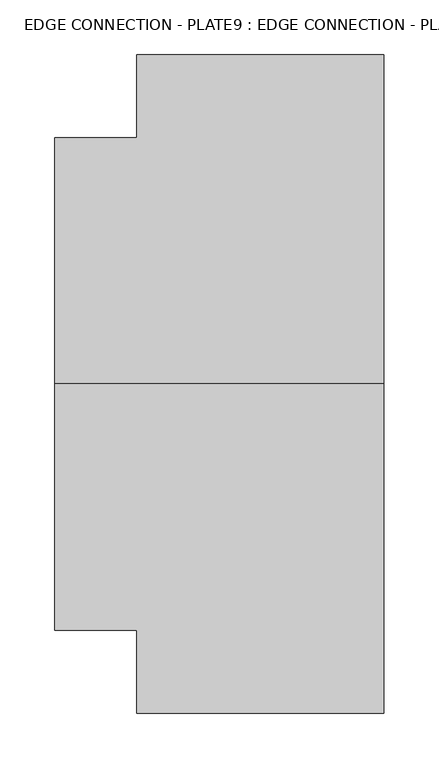
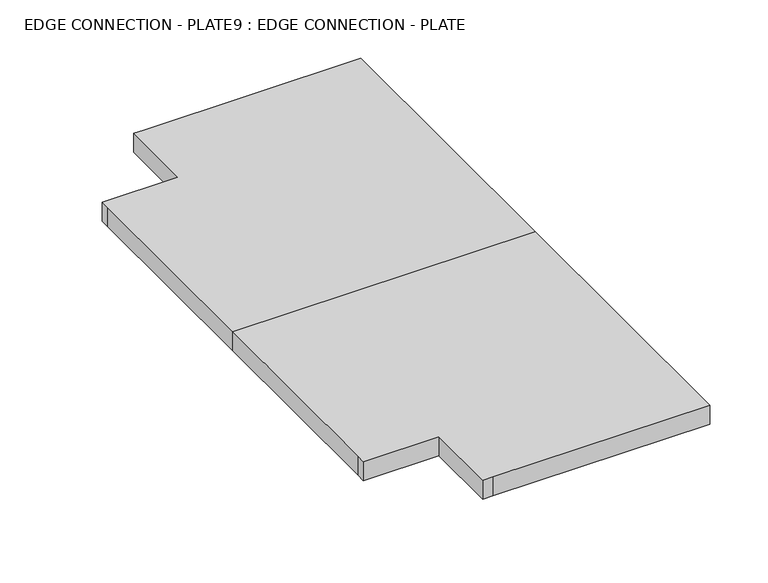
"""IFC4 building model written with IfcOpenShell, lengths in millimetres: fastener geometry, EDGE CONNECTION - PLATE9 : EDGE CONNECTION - PLATE."""

import ifcopenshell
import ifcopenshell.guid

model = None  # the IFC model being written
_history = None  # IfcOwnerHistory: only IFC2X3 demands one
_inside = {}  # id of a spatial element -> (the spatial element, [elements in it])
_under = {}  # id of a project, library or spatial element -> (it, [spatial elements below it])
_declared = {}  # id of a project -> (the project, [libraries it declares])
_typed = {}  # id of a type object -> (the type object, [elements of that type])
_made_of = {}  # id of a material, layer set ... -> (it, [elements and type objects made of it])


def new_model(schema):
    """Start an empty IFC model of exactly this schema.

    Asked for "IFC4X3", IfcOpenShell would pick the latest addendum, in which some entities
    have other attributes; the version numbers below select the first issue.
    IFC2X3 requires an IfcOwnerHistory on every rooted entity: one is made here for all.
    """
    global model, _history
    if schema == "IFC4X3":
        model = ifcopenshell.file(schema_version=(4, 3, 0, 0))
    else:
        model = ifcopenshell.file(schema=schema)
    _inside.clear()
    _under.clear()
    _declared.clear()
    _typed.clear()
    _made_of.clear()
    _history = None
    if model.schema == "IFC2X3":
        org = make("IfcOrganization", Name="unknown")
        user = make(
            "IfcPersonAndOrganization",
            ThePerson=make("IfcPerson", FamilyName="unknown"),
            TheOrganization=org,
        )
        app = make(
            "IfcApplication",
            ApplicationDeveloper=org,
            Version="unknown",
            ApplicationFullName="unknown",
            ApplicationIdentifier="unknown",
        )
        _history = make(
            "IfcOwnerHistory",
            OwningUser=user,
            OwningApplication=app,
            ChangeAction="ADDED",
            CreationDate=0,
        )
    return model


def make(cls, **values):
    """One entity of the class cls with the attributes given. An attribute that is None is left unset."""
    return model.create_entity(
        cls, **{name: value for name, value in values.items() if value is not None}
    )


def rooted(cls, **values):
    """An entity with a GlobalId (a new one), such as an element, a storey or a relation."""
    return make(cls, GlobalId=ifcopenshell.guid.new(), OwnerHistory=_history, **values)


def si_unit(unit_type, name, prefix=None):
    """IfcSIUnit, for example si_unit("LENGTHUNIT", "METRE", prefix="MILLI")."""
    return make("IfcSIUnit", UnitType=unit_type, Prefix=prefix, Name=name)


def assignment(units):
    """IfcUnitAssignment: the units of a project."""
    return None if units is None else make("IfcUnitAssignment", Units=units)


def point(xyz):
    """IfcCartesianPoint."""
    return None if xyz is None else make("IfcCartesianPoint", Coordinates=xyz)


def direction(xyz):
    """IfcDirection."""
    return None if xyz is None else make("IfcDirection", DirectionRatios=xyz)


def frame(location, z_axis=None, x_axis=None):
    """IfcAxis2Placement3D, a coordinate frame: its origin and axes. An axis left out is left unset."""
    return make(
        "IfcAxis2Placement3D",
        Location=point(location),
        Axis=direction(z_axis),
        RefDirection=direction(x_axis),
    )


def origin():
    """The frame at (0, 0, 0) with its axes left unset."""
    return frame((0.0, 0.0, 0.0))


def place(relative_to, where):
    """IfcLocalPlacement: puts the frame where relative to a parent placement (None: the world)."""
    return make(
        "IfcLocalPlacement", PlacementRelTo=relative_to, RelativePlacement=where
    )


def context(
    kind, dimensions, precision=None, world=None, true_north=None, identifier=None
):
    """IfcGeometricRepresentationContext, for example the 3D "Model" context."""
    return make(
        "IfcGeometricRepresentationContext",
        ContextIdentifier=identifier,
        ContextType=kind,
        CoordinateSpaceDimension=dimensions,
        Precision=precision,
        WorldCoordinateSystem=world,
        TrueNorth=true_north,
    )


def project(units=None, contexts=None):
    """IfcProject with its units and contexts."""
    return rooted(
        "IfcProject",
        Name="project",
        RepresentationContexts=contexts,
        UnitsInContext=assignment(units),
    )


def spatial(cls, under=None, at=None, **own):
    """A site, building, storey or space (cls), placed at a placement, below another one or the project."""
    s = rooted(cls, ObjectPlacement=at, **own)
    if under is not None:
        _under.setdefault(under.id(), (under, []))[1].append(s)
    return s


def polyline(points):
    """IfcPolyline through the points."""
    return make("IfcPolyline", Points=[point(p) for p in points])


def outline(outer, holes=None, kind="AREA"):
    """IfcArbitraryClosedProfileDef: a profile drawn as a closed curve; with holes, ...WithVoids."""
    if holes is None:
        return make("IfcArbitraryClosedProfileDef", ProfileType=kind, OuterCurve=outer)
    return make(
        "IfcArbitraryProfileDefWithVoids",
        ProfileType=kind,
        OuterCurve=outer,
        InnerCurves=holes,
    )


def extrude(swept, where, along, depth):
    """IfcExtrudedAreaSolid: the profile swept, set in the frame where, extruded along a direction by depth."""
    return make(
        "IfcExtrudedAreaSolid",
        SweptArea=swept,
        Position=where,
        ExtrudedDirection=direction(along),
        Depth=depth,
    )


def shape(context_of_items, identifier, shape_type, items):
    """IfcShapeRepresentation: the items that make up one representation, for example the "Body"."""
    return make(
        "IfcShapeRepresentation",
        ContextOfItems=context_of_items,
        RepresentationIdentifier=identifier,
        RepresentationType=shape_type,
        Items=items,
    )


def source(mapping_origin, context_of_items, identifier, shape_type, items):
    """IfcRepresentationMap: a shape defined once, which mapped items show again and again."""
    return make(
        "IfcRepresentationMap",
        MappingOrigin=mapping_origin,
        MappedRepresentation=shape(context_of_items, identifier, shape_type, items),
    )


def transform(
    local_origin,
    x_axis=None,
    y_axis=None,
    z_axis=None,
    scale=None,
    scale2=None,
    scale3=None,
    uniform=True,
):
    """IfcCartesianTransformationOperator3D, or its non-uniform kind. x_axis, y_axis, z_axis: its Axis1, 2, 3."""
    if uniform:
        return make(
            "IfcCartesianTransformationOperator3D",
            Axis1=direction(x_axis),
            Axis2=direction(y_axis),
            LocalOrigin=point(local_origin),
            Scale=scale,
            Axis3=direction(z_axis),
        )
    return make(
        "IfcCartesianTransformationOperator3DnonUniform",
        Axis1=direction(x_axis),
        Axis2=direction(y_axis),
        LocalOrigin=point(local_origin),
        Scale=scale,
        Axis3=direction(z_axis),
        Scale2=scale2,
        Scale3=scale3,
    )


def mapped(mapping_source, mapping_target):
    """IfcMappedItem: shows the shape of a source again, moved by a transform."""
    return make(
        "IfcMappedItem", MappingSource=mapping_source, MappingTarget=mapping_target
    )


def made_of(thing, what):
    """Note that an element or type object is made of a material, layer set ...; save() writes the relation."""
    if what is not None:
        _made_of.setdefault(what.id(), (what, []))[1].append(thing)
    return thing


def element(
    cls,
    number,
    at=None,
    inside=None,
    cuts=None,
    type_object=None,
    material=None,
    context=None,
    identifier="Body",
    shape_type=None,
    held_by="IfcProductDefinitionShape",
    body=None,
    shapes=None,
    **own,
):
    """One element of the class cls, such as IfcWall. Its Tag is "e" and its number.

    at: its placement. inside: the storey or other place that contains it. cuts: it is an
    opening in that element (IfcRelVoidsElement). A single representation is given by context,
    identifier, shape_type and body (its items); several are given by shapes. held_by: the class
    of the entity that holds the representations. save() writes the other relations.
    """
    e = rooted(cls, Tag="e%d" % number, ObjectPlacement=at, **own)
    if body is not None:
        shapes = [shape(context, identifier, shape_type, body)]
    if shapes is not None:
        e.Representation = make(held_by, Representations=shapes)
    if inside is not None:
        _inside.setdefault(inside.id(), (inside, []))[1].append(e)
    if cuts is not None:
        rooted(
            "IfcRelVoidsElement", RelatingBuildingElement=cuts, RelatedOpeningElement=e
        )
    if type_object is not None:
        _typed.setdefault(type_object.id(), (type_object, []))[1].append(e)
    return made_of(e, material)


def aggregate(whole, parts):
    """IfcRelAggregates: a whole, such as a stair, and the parts it consists of."""
    return rooted("IfcRelAggregates", RelatingObject=whole, RelatedObjects=parts)


def save(model, path):
    """Write the relations noted so far, then the file.

    IfcRelAggregates (storeys below a building ...), IfcRelContainedInSpatialStructure (elements
    in a storey), IfcRelDefinesByType, IfcRelAssociatesMaterial and IfcRelDeclares: one each for
    every whole, place, type object, material and project.
    """
    for whole, parts in _under.values():
        aggregate(whole, parts)
    for where, things in _inside.values():
        rooted(
            "IfcRelContainedInSpatialStructure",
            RelatedElements=things,
            RelatingStructure=where,
        )
    for kind, things in _typed.values():
        rooted("IfcRelDefinesByType", RelatedObjects=things, RelatingType=kind)
    for what, things in _made_of.values():
        rooted("IfcRelAssociatesMaterial", RelatedObjects=things, RelatingMaterial=what)
    for by, libraries in _declared.values():
        rooted("IfcRelDeclares", RelatingContext=by, RelatedDefinitions=libraries)
    model.write(path)


def edge_connection_plate9_edge_connection_plate_92328383(model_context):
    return source(origin(), model_context, "Body", "SweptSolid", [
        extrude(outline(polyline([(29700.0, 22499.5208589), (30000.0, 22499.5208589), (30000.0, 22199.5208589), (29784.862, 22199.5208589), (29774.862, 22199.5208589), (29774.862, 22275.0508589), (29700.0, 22275.0508589), (29700.0, 22285.0508589), (29700.0, 22499.5208589)])), frame((0.0, 0.0, 200.0), z_axis=(0.0, 0.0, 1.0), x_axis=(1.0, 0.0, 0.0)), (0.0, 0.0, 1.0), 20.0),
        extrude(outline(polyline([(29700.0, 22499.5208589), (29700.0, 22713.9908589), (29700.0, 22723.9908589), (29774.862, 22723.9908589), (29774.862, 22799.5208589), (29784.862, 22799.5208589), (30000.0, 22799.5208589), (30000.0, 22499.5208589), (29700.0, 22499.5208589)])), frame((0.0, 0.0, 200.0), z_axis=(0.0, 0.0, 1.0), x_axis=(1.0, 0.0, 0.0)), (0.0, 0.0, 1.0), 20.0),
    ])


if __name__ == "__main__":
    model = new_model("IFC4")
    model_context = context("Model", 3, world=origin())
    ifc_project = project(units=[si_unit("LENGTHUNIT", "METRE", prefix="MILLI")], contexts=[model_context])
    site = spatial("IfcSite", under=ifc_project)
    building = spatial("IfcBuilding", under=site)
    placement = place(None, origin())
    edge_connection_plate9_edge_connection_plate_shape = edge_connection_plate9_edge_connection_plate_92328383(model_context)
    element("IfcFastener", 1, ObjectType="EDGE CONNECTION - PLATE9 : EDGE CONNECTION - PLATE", at=placement, inside=building, context=model_context, shape_type="MappedRepresentation", body=[
        mapped(edge_connection_plate9_edge_connection_plate_shape, transform((0.0, 0.0, 0.0), x_axis=(1.0, 0.0, 0.0), y_axis=(0.0, 1.0, 0.0), z_axis=(0.0, 0.0, 1.0))),
    ])
    save(model, "model.ifc")
